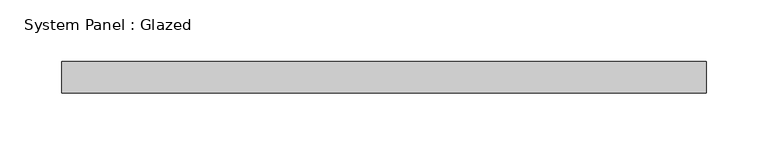
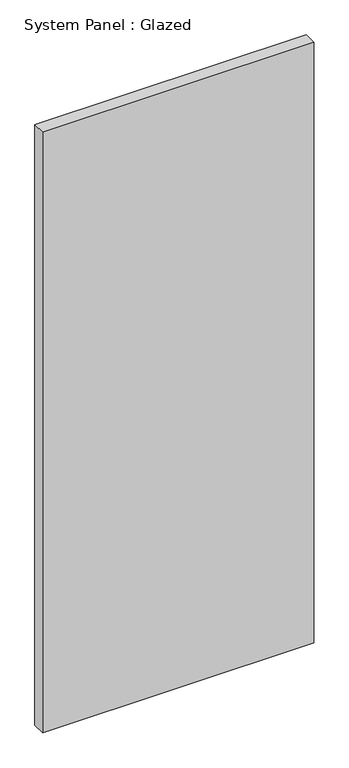
"""IFC4 building model written with IfcOpenShell, lengths in millimetres: plate geometry, System Panel : Glazed."""

import ifcopenshell
import ifcopenshell.guid

model = None  # the IFC model being written
_history = None  # IfcOwnerHistory: only IFC2X3 demands one
_inside = {}  # id of a spatial element -> (the spatial element, [elements in it])
_under = {}  # id of a project, library or spatial element -> (it, [spatial elements below it])
_declared = {}  # id of a project -> (the project, [libraries it declares])
_typed = {}  # id of a type object -> (the type object, [elements of that type])
_made_of = {}  # id of a material, layer set ... -> (it, [elements and type objects made of it])


def new_model(schema):
    """Start an empty IFC model of exactly this schema.

    Asked for "IFC4X3", IfcOpenShell would pick the latest addendum, in which some entities
    have other attributes; the version numbers below select the first issue.
    IFC2X3 requires an IfcOwnerHistory on every rooted entity: one is made here for all.
    """
    global model, _history
    if schema == "IFC4X3":
        model = ifcopenshell.file(schema_version=(4, 3, 0, 0))
    else:
        model = ifcopenshell.file(schema=schema)
    _inside.clear()
    _under.clear()
    _declared.clear()
    _typed.clear()
    _made_of.clear()
    _history = None
    if model.schema == "IFC2X3":
        org = make("IfcOrganization", Name="unknown")
        user = make(
            "IfcPersonAndOrganization",
            ThePerson=make("IfcPerson", FamilyName="unknown"),
            TheOrganization=org,
        )
        app = make(
            "IfcApplication",
            ApplicationDeveloper=org,
            Version="unknown",
            ApplicationFullName="unknown",
            ApplicationIdentifier="unknown",
        )
        _history = make(
            "IfcOwnerHistory",
            OwningUser=user,
            OwningApplication=app,
            ChangeAction="ADDED",
            CreationDate=0,
        )
    return model


def make(cls, **values):
    """One entity of the class cls with the attributes given. An attribute that is None is left unset."""
    return model.create_entity(
        cls, **{name: value for name, value in values.items() if value is not None}
    )


def rooted(cls, **values):
    """An entity with a GlobalId (a new one), such as an element, a storey or a relation."""
    return make(cls, GlobalId=ifcopenshell.guid.new(), OwnerHistory=_history, **values)


def si_unit(unit_type, name, prefix=None):
    """IfcSIUnit, for example si_unit("LENGTHUNIT", "METRE", prefix="MILLI")."""
    return make("IfcSIUnit", UnitType=unit_type, Prefix=prefix, Name=name)


def assignment(units):
    """IfcUnitAssignment: the units of a project."""
    return None if units is None else make("IfcUnitAssignment", Units=units)


def point(xyz):
    """IfcCartesianPoint."""
    return None if xyz is None else make("IfcCartesianPoint", Coordinates=xyz)


def direction(xyz):
    """IfcDirection."""
    return None if xyz is None else make("IfcDirection", DirectionRatios=xyz)


def frame(location, z_axis=None, x_axis=None):
    """IfcAxis2Placement3D, a coordinate frame: its origin and axes. An axis left out is left unset."""
    return make(
        "IfcAxis2Placement3D",
        Location=point(location),
        Axis=direction(z_axis),
        RefDirection=direction(x_axis),
    )


def origin():
    """The frame at (0, 0, 0) with its axes left unset."""
    return frame((0.0, 0.0, 0.0))


def origin_with_axes():
    """The frame at (0, 0, 0) with the z axis (0, 0, 1) and the x axis (1, 0, 0) written out."""
    return frame((0.0, 0.0, 0.0), z_axis=(0.0, 0.0, 1.0), x_axis=(1.0, 0.0, 0.0))


def place(relative_to, where):
    """IfcLocalPlacement: puts the frame where relative to a parent placement (None: the world)."""
    return make(
        "IfcLocalPlacement", PlacementRelTo=relative_to, RelativePlacement=where
    )


def context(
    kind, dimensions, precision=None, world=None, true_north=None, identifier=None
):
    """IfcGeometricRepresentationContext, for example the 3D "Model" context."""
    return make(
        "IfcGeometricRepresentationContext",
        ContextIdentifier=identifier,
        ContextType=kind,
        CoordinateSpaceDimension=dimensions,
        Precision=precision,
        WorldCoordinateSystem=world,
        TrueNorth=true_north,
    )


def project(units=None, contexts=None):
    """IfcProject with its units and contexts."""
    return rooted(
        "IfcProject",
        Name="project",
        RepresentationContexts=contexts,
        UnitsInContext=assignment(units),
    )


def spatial(cls, under=None, at=None, **own):
    """A site, building, storey or space (cls), placed at a placement, below another one or the project."""
    s = rooted(cls, ObjectPlacement=at, **own)
    if under is not None:
        _under.setdefault(under.id(), (under, []))[1].append(s)
    return s


def polyline(points):
    """IfcPolyline through the points."""
    return make("IfcPolyline", Points=[point(p) for p in points])


def outline(outer, holes=None, kind="AREA"):
    """IfcArbitraryClosedProfileDef: a profile drawn as a closed curve; with holes, ...WithVoids."""
    if holes is None:
        return make("IfcArbitraryClosedProfileDef", ProfileType=kind, OuterCurve=outer)
    return make(
        "IfcArbitraryProfileDefWithVoids",
        ProfileType=kind,
        OuterCurve=outer,
        InnerCurves=holes,
    )


def extrude(swept, where, along, depth):
    """IfcExtrudedAreaSolid: the profile swept, set in the frame where, extruded along a direction by depth."""
    return make(
        "IfcExtrudedAreaSolid",
        SweptArea=swept,
        Position=where,
        ExtrudedDirection=direction(along),
        Depth=depth,
    )


def shape(context_of_items, identifier, shape_type, items):
    """IfcShapeRepresentation: the items that make up one representation, for example the "Body"."""
    return make(
        "IfcShapeRepresentation",
        ContextOfItems=context_of_items,
        RepresentationIdentifier=identifier,
        RepresentationType=shape_type,
        Items=items,
    )


def source(mapping_origin, context_of_items, identifier, shape_type, items):
    """IfcRepresentationMap: a shape defined once, which mapped items show again and again."""
    return make(
        "IfcRepresentationMap",
        MappingOrigin=mapping_origin,
        MappedRepresentation=shape(context_of_items, identifier, shape_type, items),
    )


def transform(
    local_origin,
    x_axis=None,
    y_axis=None,
    z_axis=None,
    scale=None,
    scale2=None,
    scale3=None,
    uniform=True,
):
    """IfcCartesianTransformationOperator3D, or its non-uniform kind. x_axis, y_axis, z_axis: its Axis1, 2, 3."""
    if uniform:
        return make(
            "IfcCartesianTransformationOperator3D",
            Axis1=direction(x_axis),
            Axis2=direction(y_axis),
            LocalOrigin=point(local_origin),
            Scale=scale,
            Axis3=direction(z_axis),
        )
    return make(
        "IfcCartesianTransformationOperator3DnonUniform",
        Axis1=direction(x_axis),
        Axis2=direction(y_axis),
        LocalOrigin=point(local_origin),
        Scale=scale,
        Axis3=direction(z_axis),
        Scale2=scale2,
        Scale3=scale3,
    )


def mapped(mapping_source, mapping_target):
    """IfcMappedItem: shows the shape of a source again, moved by a transform."""
    return make(
        "IfcMappedItem", MappingSource=mapping_source, MappingTarget=mapping_target
    )


def made_of(thing, what):
    """Note that an element or type object is made of a material, layer set ...; save() writes the relation."""
    if what is not None:
        _made_of.setdefault(what.id(), (what, []))[1].append(thing)
    return thing


def element(
    cls,
    number,
    at=None,
    inside=None,
    cuts=None,
    type_object=None,
    material=None,
    context=None,
    identifier="Body",
    shape_type=None,
    held_by="IfcProductDefinitionShape",
    body=None,
    shapes=None,
    **own,
):
    """One element of the class cls, such as IfcWall. Its Tag is "e" and its number.

    at: its placement. inside: the storey or other place that contains it. cuts: it is an
    opening in that element (IfcRelVoidsElement). A single representation is given by context,
    identifier, shape_type and body (its items); several are given by shapes. held_by: the class
    of the entity that holds the representations. save() writes the other relations.
    """
    e = rooted(cls, Tag="e%d" % number, ObjectPlacement=at, **own)
    if body is not None:
        shapes = [shape(context, identifier, shape_type, body)]
    if shapes is not None:
        e.Representation = make(held_by, Representations=shapes)
    if inside is not None:
        _inside.setdefault(inside.id(), (inside, []))[1].append(e)
    if cuts is not None:
        rooted(
            "IfcRelVoidsElement", RelatingBuildingElement=cuts, RelatedOpeningElement=e
        )
    if type_object is not None:
        _typed.setdefault(type_object.id(), (type_object, []))[1].append(e)
    return made_of(e, material)


def aggregate(whole, parts):
    """IfcRelAggregates: a whole, such as a stair, and the parts it consists of."""
    return rooted("IfcRelAggregates", RelatingObject=whole, RelatedObjects=parts)


def save(model, path):
    """Write the relations noted so far, then the file.

    IfcRelAggregates (storeys below a building ...), IfcRelContainedInSpatialStructure (elements
    in a storey), IfcRelDefinesByType, IfcRelAssociatesMaterial and IfcRelDeclares: one each for
    every whole, place, type object, material and project.
    """
    for whole, parts in _under.values():
        aggregate(whole, parts)
    for where, things in _inside.values():
        rooted(
            "IfcRelContainedInSpatialStructure",
            RelatedElements=things,
            RelatingStructure=where,
        )
    for kind, things in _typed.values():
        rooted("IfcRelDefinesByType", RelatedObjects=things, RelatingType=kind)
    for what, things in _made_of.values():
        rooted("IfcRelAssociatesMaterial", RelatedObjects=things, RelatingMaterial=what)
    for by, libraries in _declared.values():
        rooted("IfcRelDeclares", RelatingContext=by, RelatedDefinitions=libraries)
    model.write(path)


def system_panel_glazed_b4adc3fa(model_context):
    return source(origin(), model_context, "Body", "SweptSolid", [
        extrude(outline(polyline([(260.35, 19.05), (-260.35, 19.05), (-260.35, 44.45), (260.35, 44.45), (260.35, 19.05)])), origin_with_axes(), (0.0, 0.0, 1.0), 1219.2),
    ])


if __name__ == "__main__":
    model = new_model("IFC4")
    model_context = context("Model", 3, world=origin())
    ifc_project = project(units=[si_unit("LENGTHUNIT", "METRE", prefix="MILLI")], contexts=[model_context])
    site = spatial("IfcSite", under=ifc_project)
    building = spatial("IfcBuilding", under=site)
    placement = place(None, origin())
    system_panel_glazed_shape = system_panel_glazed_b4adc3fa(model_context)
    element("IfcPlate", 1, ObjectType="System Panel : Glazed", at=placement, inside=building, context=model_context, shape_type="MappedRepresentation", body=[
        mapped(system_panel_glazed_shape, transform((0.0, 0.0, 0.0), x_axis=(1.0, 0.0, 0.0), y_axis=(0.0, 1.0, 0.0), z_axis=(0.0, 0.0, 1.0))),
    ])
    save(model, "model.ifc")

# Revit data of these elements
# Element 1 (IfcPlate, "System Panel : Glazed")
#   Materials on its faces: "Glass"
# Materials
#   "Glass": class "Glass", colour RGB 0 128 192, transparency 0.75
